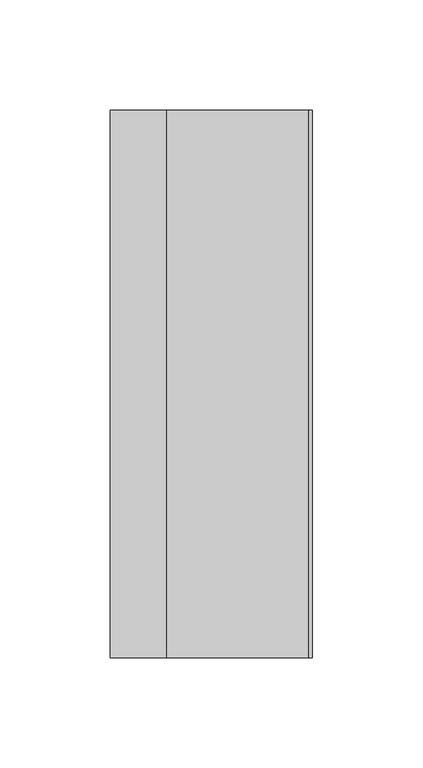
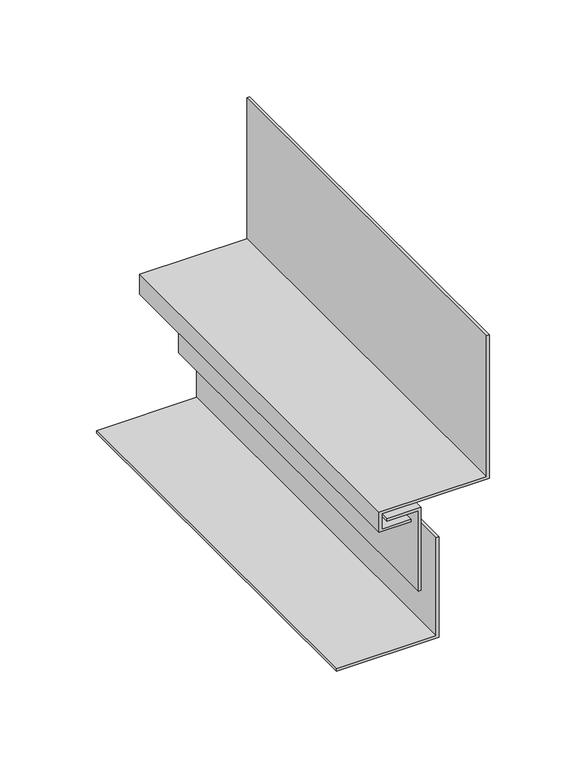
"""IFC4 building model written with IfcOpenShell, lengths in millimetres: proxy geometry, Generic Models 2:Generic Models 2:310765:Generic Models 2:310765 : Generic Models 2:Generic Models 2:310765:80 : Generic Models 2:Generic Models 2:310765:Generic Models 2:310765 : Generic Models 2:Generic Models 2:310765:300385."""

import ifcopenshell
import ifcopenshell.guid

model = None  # the IFC model being written
_history = None  # IfcOwnerHistory: only IFC2X3 demands one
_inside = {}  # id of a spatial element -> (the spatial element, [elements in it])
_under = {}  # id of a project, library or spatial element -> (it, [spatial elements below it])
_declared = {}  # id of a project -> (the project, [libraries it declares])
_typed = {}  # id of a type object -> (the type object, [elements of that type])
_made_of = {}  # id of a material, layer set ... -> (it, [elements and type objects made of it])


def new_model(schema):
    """Start an empty IFC model of exactly this schema.

    Asked for "IFC4X3", IfcOpenShell would pick the latest addendum, in which some entities
    have other attributes; the version numbers below select the first issue.
    IFC2X3 requires an IfcOwnerHistory on every rooted entity: one is made here for all.
    """
    global model, _history
    if schema == "IFC4X3":
        model = ifcopenshell.file(schema_version=(4, 3, 0, 0))
    else:
        model = ifcopenshell.file(schema=schema)
    _inside.clear()
    _under.clear()
    _declared.clear()
    _typed.clear()
    _made_of.clear()
    _history = None
    if model.schema == "IFC2X3":
        org = make("IfcOrganization", Name="unknown")
        user = make(
            "IfcPersonAndOrganization",
            ThePerson=make("IfcPerson", FamilyName="unknown"),
            TheOrganization=org,
        )
        app = make(
            "IfcApplication",
            ApplicationDeveloper=org,
            Version="unknown",
            ApplicationFullName="unknown",
            ApplicationIdentifier="unknown",
        )
        _history = make(
            "IfcOwnerHistory",
            OwningUser=user,
            OwningApplication=app,
            ChangeAction="ADDED",
            CreationDate=0,
        )
    return model


def make(cls, **values):
    """One entity of the class cls with the attributes given. An attribute that is None is left unset."""
    return model.create_entity(
        cls, **{name: value for name, value in values.items() if value is not None}
    )


def rooted(cls, **values):
    """An entity with a GlobalId (a new one), such as an element, a storey or a relation."""
    return make(cls, GlobalId=ifcopenshell.guid.new(), OwnerHistory=_history, **values)


def si_unit(unit_type, name, prefix=None):
    """IfcSIUnit, for example si_unit("LENGTHUNIT", "METRE", prefix="MILLI")."""
    return make("IfcSIUnit", UnitType=unit_type, Prefix=prefix, Name=name)


def assignment(units):
    """IfcUnitAssignment: the units of a project."""
    return None if units is None else make("IfcUnitAssignment", Units=units)


def point(xyz):
    """IfcCartesianPoint."""
    return None if xyz is None else make("IfcCartesianPoint", Coordinates=xyz)


def direction(xyz):
    """IfcDirection."""
    return None if xyz is None else make("IfcDirection", DirectionRatios=xyz)


def frame(location, z_axis=None, x_axis=None):
    """IfcAxis2Placement3D, a coordinate frame: its origin and axes. An axis left out is left unset."""
    return make(
        "IfcAxis2Placement3D",
        Location=point(location),
        Axis=direction(z_axis),
        RefDirection=direction(x_axis),
    )


def origin():
    """The frame at (0, 0, 0) with its axes left unset."""
    return frame((0.0, 0.0, 0.0))


def place(relative_to, where):
    """IfcLocalPlacement: puts the frame where relative to a parent placement (None: the world)."""
    return make(
        "IfcLocalPlacement", PlacementRelTo=relative_to, RelativePlacement=where
    )


def context(
    kind, dimensions, precision=None, world=None, true_north=None, identifier=None
):
    """IfcGeometricRepresentationContext, for example the 3D "Model" context."""
    return make(
        "IfcGeometricRepresentationContext",
        ContextIdentifier=identifier,
        ContextType=kind,
        CoordinateSpaceDimension=dimensions,
        Precision=precision,
        WorldCoordinateSystem=world,
        TrueNorth=true_north,
    )


def project(units=None, contexts=None):
    """IfcProject with its units and contexts."""
    return rooted(
        "IfcProject",
        Name="project",
        RepresentationContexts=contexts,
        UnitsInContext=assignment(units),
    )


def spatial(cls, under=None, at=None, **own):
    """A site, building, storey or space (cls), placed at a placement, below another one or the project."""
    s = rooted(cls, ObjectPlacement=at, **own)
    if under is not None:
        _under.setdefault(under.id(), (under, []))[1].append(s)
    return s


def polyline(points):
    """IfcPolyline through the points."""
    return make("IfcPolyline", Points=[point(p) for p in points])


def outline(outer, holes=None, kind="AREA"):
    """IfcArbitraryClosedProfileDef: a profile drawn as a closed curve; with holes, ...WithVoids."""
    if holes is None:
        return make("IfcArbitraryClosedProfileDef", ProfileType=kind, OuterCurve=outer)
    return make(
        "IfcArbitraryProfileDefWithVoids",
        ProfileType=kind,
        OuterCurve=outer,
        InnerCurves=holes,
    )


def extrude(swept, where, along, depth):
    """IfcExtrudedAreaSolid: the profile swept, set in the frame where, extruded along a direction by depth."""
    return make(
        "IfcExtrudedAreaSolid",
        SweptArea=swept,
        Position=where,
        ExtrudedDirection=direction(along),
        Depth=depth,
    )


def shape(context_of_items, identifier, shape_type, items):
    """IfcShapeRepresentation: the items that make up one representation, for example the "Body"."""
    return make(
        "IfcShapeRepresentation",
        ContextOfItems=context_of_items,
        RepresentationIdentifier=identifier,
        RepresentationType=shape_type,
        Items=items,
    )


def source(mapping_origin, context_of_items, identifier, shape_type, items):
    """IfcRepresentationMap: a shape defined once, which mapped items show again and again."""
    return make(
        "IfcRepresentationMap",
        MappingOrigin=mapping_origin,
        MappedRepresentation=shape(context_of_items, identifier, shape_type, items),
    )


def transform(
    local_origin,
    x_axis=None,
    y_axis=None,
    z_axis=None,
    scale=None,
    scale2=None,
    scale3=None,
    uniform=True,
):
    """IfcCartesianTransformationOperator3D, or its non-uniform kind. x_axis, y_axis, z_axis: its Axis1, 2, 3."""
    if uniform:
        return make(
            "IfcCartesianTransformationOperator3D",
            Axis1=direction(x_axis),
            Axis2=direction(y_axis),
            LocalOrigin=point(local_origin),
            Scale=scale,
            Axis3=direction(z_axis),
        )
    return make(
        "IfcCartesianTransformationOperator3DnonUniform",
        Axis1=direction(x_axis),
        Axis2=direction(y_axis),
        LocalOrigin=point(local_origin),
        Scale=scale,
        Axis3=direction(z_axis),
        Scale2=scale2,
        Scale3=scale3,
    )


def mapped(mapping_source, mapping_target):
    """IfcMappedItem: shows the shape of a source again, moved by a transform."""
    return make(
        "IfcMappedItem", MappingSource=mapping_source, MappingTarget=mapping_target
    )


def made_of(thing, what):
    """Note that an element or type object is made of a material, layer set ...; save() writes the relation."""
    if what is not None:
        _made_of.setdefault(what.id(), (what, []))[1].append(thing)
    return thing


def element(
    cls,
    number,
    at=None,
    inside=None,
    cuts=None,
    type_object=None,
    material=None,
    context=None,
    identifier="Body",
    shape_type=None,
    held_by="IfcProductDefinitionShape",
    body=None,
    shapes=None,
    **own,
):
    """One element of the class cls, such as IfcWall. Its Tag is "e" and its number.

    at: its placement. inside: the storey or other place that contains it. cuts: it is an
    opening in that element (IfcRelVoidsElement). A single representation is given by context,
    identifier, shape_type and body (its items); several are given by shapes. held_by: the class
    of the entity that holds the representations. save() writes the other relations.
    """
    e = rooted(cls, Tag="e%d" % number, ObjectPlacement=at, **own)
    if body is not None:
        shapes = [shape(context, identifier, shape_type, body)]
    if shapes is not None:
        e.Representation = make(held_by, Representations=shapes)
    if inside is not None:
        _inside.setdefault(inside.id(), (inside, []))[1].append(e)
    if cuts is not None:
        rooted(
            "IfcRelVoidsElement", RelatingBuildingElement=cuts, RelatedOpeningElement=e
        )
    if type_object is not None:
        _typed.setdefault(type_object.id(), (type_object, []))[1].append(e)
    return made_of(e, material)


def aggregate(whole, parts):
    """IfcRelAggregates: a whole, such as a stair, and the parts it consists of."""
    return rooted("IfcRelAggregates", RelatingObject=whole, RelatedObjects=parts)


def save(model, path):
    """Write the relations noted so far, then the file.

    IfcRelAggregates (storeys below a building ...), IfcRelContainedInSpatialStructure (elements
    in a storey), IfcRelDefinesByType, IfcRelAssociatesMaterial and IfcRelDeclares: one each for
    every whole, place, type object, material and project.
    """
    for whole, parts in _under.values():
        aggregate(whole, parts)
    for where, things in _inside.values():
        rooted(
            "IfcRelContainedInSpatialStructure",
            RelatedElements=things,
            RelatingStructure=where,
        )
    for kind, things in _typed.values():
        rooted("IfcRelDefinesByType", RelatedObjects=things, RelatingType=kind)
    for what, things in _made_of.values():
        rooted("IfcRelAssociatesMaterial", RelatedObjects=things, RelatingMaterial=what)
    for by, libraries in _declared.values():
        rooted("IfcRelDeclares", RelatingContext=by, RelatedDefinitions=libraries)
    model.write(path)


def generic_models_1e1107b9(model_context):
    return source(origin(), model_context, "Body", "SweptSolid", [
        extrude(outline(polyline([(4026.4869619, 560370.4242239), (4116.9744619, 560370.4242239), (4116.9744619, 560368.8367239), (4028.0744619, 560368.8367239), (4028.0744619, 560304.6791598), (4015.3744619, 560304.6791598), (4015.3744619, 560323.7291598), (4016.9619619, 560323.7291598), (4016.9619619, 560306.2666598), (4026.4869619, 560306.2666598), (4026.4869619, 560370.4242239)])), frame((0.0, -579011.8786724, 0.0), z_axis=(0.0, 1.0, 0.0), x_axis=(0.0, 0.0, 1.0)), (0.0, 0.0, 1.0), 247.8463739),
        extrude(outline(polyline([(4020.9307119, 560328.0732928), (3970.1307119, 560328.0732928), (3970.1307119, 560329.6607928), (4022.5182119, 560329.6607928), (4022.5182119, 560309.2041611), (4020.9307119, 560309.2041611), (4020.9307119, 560328.0732928)])), frame((0.0, -579011.8786724, 0.0), z_axis=(0.0, 1.0, 0.0), x_axis=(0.0, 0.0, 1.0)), (0.0, 0.0, 1.0), 247.8463739),
        extrude(outline(polyline([(3936.7932119, 560340.2617239), (4000.2932119, 560340.2617239), (4000.2932119, 560338.6742239), (3938.3807119, 560338.6742239), (3938.3807119, 560279.0416611), (3936.7932119, 560279.0416611), (3936.7932119, 560340.2617239)])), frame((0.0, -579011.8786724, 0.0), z_axis=(0.0, 1.0, 0.0), x_axis=(0.0, 0.0, 1.0)), (0.0, 0.0, 1.0), 247.8463739),
    ])


if __name__ == "__main__":
    model = new_model("IFC4")
    model_context = context("Model", 3, world=origin())
    ifc_project = project(units=[si_unit("LENGTHUNIT", "METRE", prefix="MILLI")], contexts=[model_context])
    site = spatial("IfcSite", under=ifc_project)
    building = spatial("IfcBuilding", under=site)
    placement = place(None, origin())
    generic_models_shape = generic_models_1e1107b9(model_context)
    element("IfcBuildingElementProxy", 1, Name="Generic Models 2:Generic Models 2:310765:Generic Models 2:310765 : Generic Models 2:Generic Models 2:310765:80 : Generic Models 2:Generic Models 2:310765:Generic Models 2:310765 : Generic Models 2:Generic Models 2:310765:300385", ObjectType="Generic Models 2:Generic Models 2:310765:Generic Models 2:310765 : Generic Models 2:Generic Models 2:310765:80 : Generic Models 2:Generic Models 2:310765:Generic Models 2:310765 : Generic Models 2:Generic Models 2:310765:300385", at=placement, inside=building, context=model_context, shape_type="MappedRepresentation", body=[
        mapped(generic_models_shape, transform((0.0, 0.0, 0.0), x_axis=(1.0, 0.0, 0.0), y_axis=(0.0, 1.0, 0.0), z_axis=(0.0, 0.0, 1.0))),
    ])
    save(model, "model.ifc")

# Revit data of these elements
# Type "Generic Models 2:Generic Models 2:310765:Generic Models 2:310765 : Generic Models 2:Generic Models 2:310765:80 : Generic Models 2:Generic Models 2:310765:Generic Models 2:310765 : Generic Models 2:Generic Models 2:310765:300385"
#   NameOverride = "Generic Models 2:Generic Models 2:310765:Generic Models 2:310765 : Generic Models 2:Generic Models 2:310765:300385"
#   ObjectTypeOverride = "Generic Models 2:310765 : Generic Models 2:Generic Models 2:310765"
#   Reference = "Generic Models 2"
#   Tag = "300385"
# Element 1 (IfcBuildingElementProxy, "Generic Models 2:Generic Models 2:310765:Generic Models 2:310765 : Generic Models 2:Generic Models 2:310765:80 : Generic Models 2:Generic Models 2:310765:Generic Models 2:310765 : Generic Models 2:Generic Models 2:310765:300385")
#   Materials on its faces: "BRAKE METAL COUNTERFLASHING"
# Materials
#   "BRAKE METAL COUNTERFLASHING": class "Unassigned", colour RGB 182 182 182, transparency 0, Cost = 0
